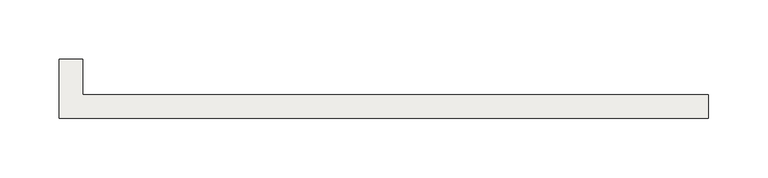
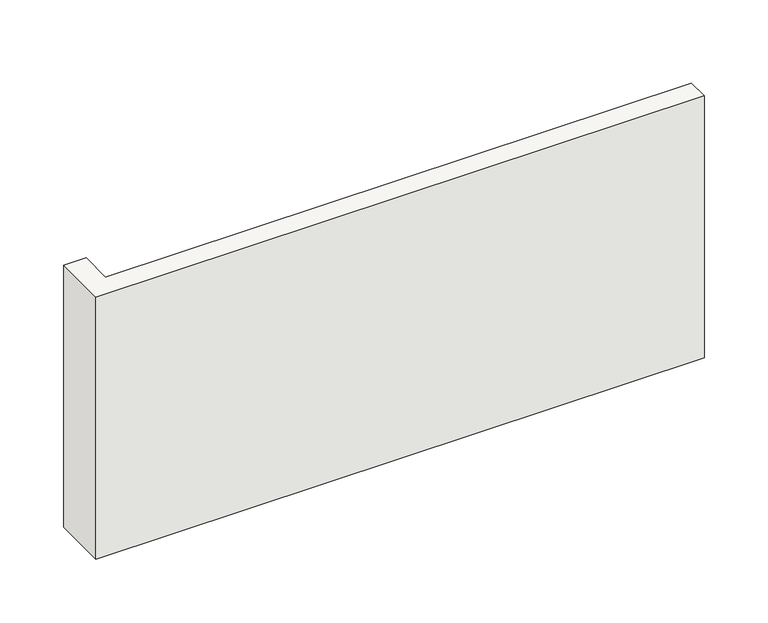
"""IFC4 building model written with IfcOpenShell, lengths in millimetres: slab geometry, FECHAMENTO DECK DE MADEIRA - PATAMAR ENTRADA1 : FECHAMENTO DECK DE MADEIRA - PATAMAR ENTRADA."""

from ifc_helpers import new_model, si_unit, frame, origin, place, context, project, spatial, polyline, outline, extrude, source, transform, mapped, element, save


def slab_4ab7dbbf(model_context):
    return source(origin(), model_context, "Body", "SweptSolid", [
        extrude(outline(polyline([(-6660.281307, -475.5699847), (-6660.281307, -495.5699847), (-7209.281307, -495.5699847), (-7209.281307, -445.5699847), (-7189.281307, -445.5699847), (-7189.281307, -475.5699847), (-6660.281307, -475.5699847)])), frame((0.0, 0.0, 80.0), z_axis=(0.0, 0.0, 1.0), x_axis=(1.0, 0.0, 0.0)), (0.0, 0.0, 1.0), 250.0),
    ])


if __name__ == "__main__":
    model = new_model("IFC4")
    model_context = context("Model", 3, world=origin())
    ifc_project = project(units=[si_unit("LENGTHUNIT", "METRE", prefix="MILLI")], contexts=[model_context])
    site = spatial("IfcSite", under=ifc_project)
    building = spatial("IfcBuilding", under=site)
    placement = place(None, origin())
    slab_shape = slab_4ab7dbbf(model_context)
    element("IfcSlab", 1, ObjectType="FECHAMENTO DECK DE MADEIRA - PATAMAR ENTRADA1 : FECHAMENTO DECK DE MADEIRA - PATAMAR ENTRADA", at=placement, inside=building, context=model_context, shape_type="MappedRepresentation", body=[
        mapped(slab_shape, transform((0.0, 0.0, 0.0), x_axis=(1.0, 0.0, 0.0), y_axis=(0.0, 1.0, 0.0), z_axis=(0.0, 0.0, 1.0))),
    ])
    save(model, "model.ifc")

# Revit data of these elements
# Element 1 (IfcSlab, "FECHAMENTO DECK DE MADEIRA - PATAMAR ENTRADA1 : FECHAMENTO DECK DE MADEIRA - PATAMAR ENTRADA")
#   Materials on its faces: ".DECK DE MADEIRA LONGITUDINAL"
# Materials
#   ".DECK DE MADEIRA LONGITUDINAL": class ".CC_MADEIRA REVEST.", colour RGB 169 114 85, transparency 0, Description = "Deck de madeira", Cost = 0
